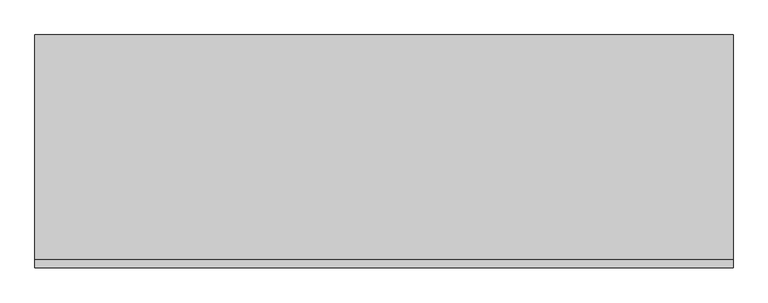
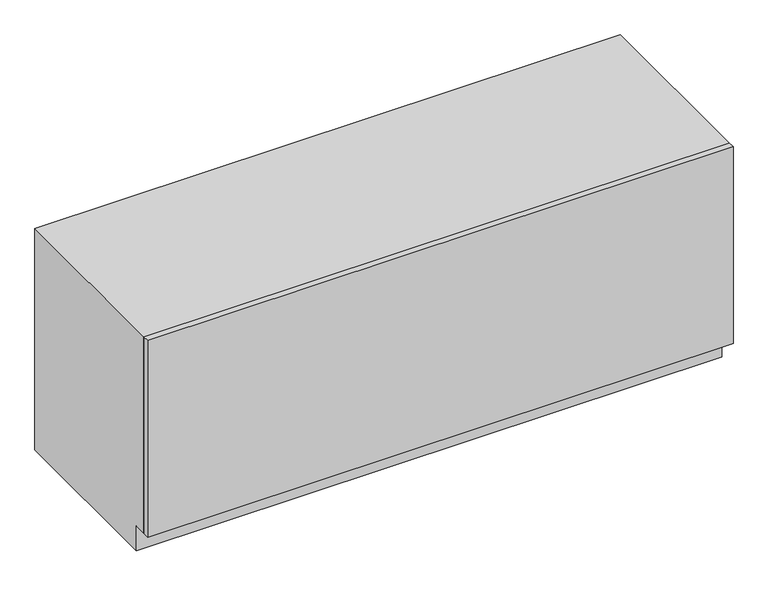
"""IFC4 building model written with IfcOpenShell, lengths in millimetres: furniture geometry, OD_CW_Base Cabinet : OD_CW_Base Cabinet."""

from ifc_helpers import new_model, si_unit, frame, origin, place, context, project, spatial, polyline, outline, extrude, source, transform, mapped, element, save


def furniture_2af7cf50(model_context):
    return source(origin(), model_context, "Body", "SweptSolid", [
        extrude(outline(polyline([(18.7377049, -127.0), (2304.7377049, -127.0), (2304.7377049, -152.4), (18.7377049, -152.4), (18.7377049, -127.0)])), frame((0.0, 0.0, 101.6), z_axis=(0.0, 0.0, 1.0), x_axis=(1.0, 0.0, 0.0)), (0.0, 0.0, 1.0), 812.8),
        extrude(outline(polyline([(-127.0, 914.4), (609.6, 914.4), (609.6, 0.0), (-76.2, 0.0), (-76.2, 101.6), (-127.0, 101.6), (-127.0, 914.4)])), frame((18.7377049, 0.0, 0.0), z_axis=(1.0, 0.0, 0.0), x_axis=(0.0, 1.0, 0.0)), (0.0, 0.0, 1.0), 2286.0),
    ])


if __name__ == "__main__":
    model = new_model("IFC4")
    model_context = context("Model", 3, world=origin())
    ifc_project = project(units=[si_unit("LENGTHUNIT", "METRE", prefix="MILLI")], contexts=[model_context])
    site = spatial("IfcSite", under=ifc_project)
    building = spatial("IfcBuilding", under=site)
    placement = place(None, origin())
    furniture_shape = furniture_2af7cf50(model_context)
    element("IfcFurniture", 1, ObjectType="OD_CW_Base Cabinet : OD_CW_Base Cabinet", at=placement, inside=building, context=model_context, shape_type="MappedRepresentation", body=[
        mapped(furniture_shape, transform((0.0, 0.0, 0.0), x_axis=(1.0, 0.0, 0.0), y_axis=(0.0, 1.0, 0.0), z_axis=(0.0, 0.0, 1.0))),
    ])
    save(model, "model.ifc")

# Revit data of these elements
# Type "OD_CW_Base Cabinet : OD_CW_Base Cabinet"
#   OD_CW_Width [instance default] = 2' - 10"
#   OD_CW_Length [instance default] = 8' - 0"
#   OD_CW_Height [instance default] = 2' - 3"
#   Depth = 2' - 0"
#   Height = 3' - 0"
#   Width = 4' - 0"
#   OD_CW_Material_Front Panel [instance default] = none
#   OD_CW_Material_Body [instance default] = none
# Element 1 (IfcFurniture, "OD_CW_Base Cabinet : OD_CW_Base Cabinet")
#   OD_CW_Width = 2' - 6"
#   OD_CW_Length = 7' - 6"
#   OD_CW_Height = 3' - 0"
#   OD_CW_Material_Body = PREP TABLE
#   Materials on its faces: "PREP TABLE", "CASEWORK"
# Materials
#   "PREP TABLE": class "Generic", colour RGB 187 187 187, transparency 0, Cost = 0
#   "CASEWORK": class "Generic", colour RGB 181 181 181, transparency 0, Cost = 0
